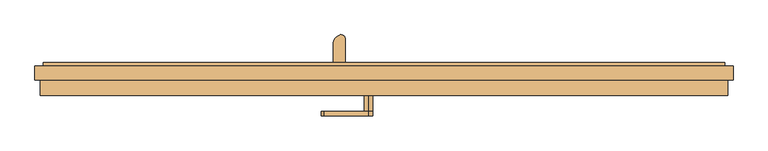
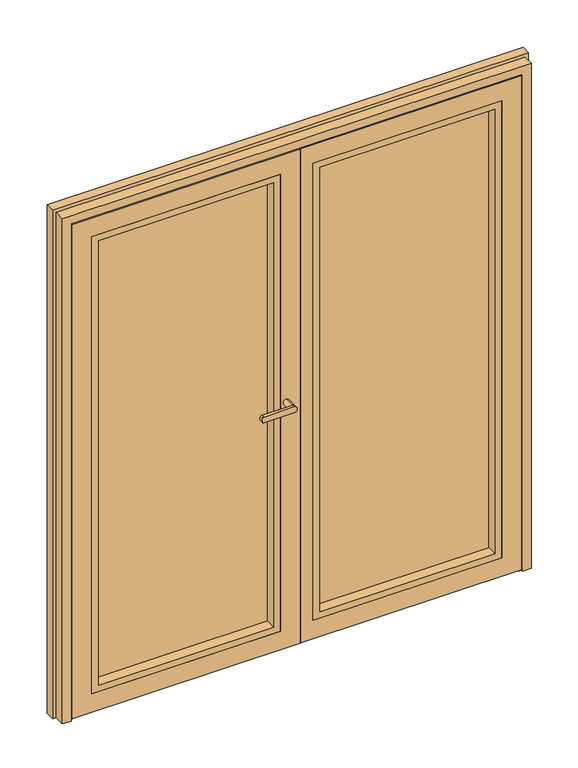
"""IFC4 building model written with IfcOpenShell, lengths in millimetres: door geometry, Schueco_FWS_ADS-90-SI_inw_Family-02 : FWS SI insert unit."""

import ifcopenshell
import ifcopenshell.guid

model = None  # the IFC model being written
_history = None  # IfcOwnerHistory: only IFC2X3 demands one
_inside = {}  # id of a spatial element -> (the spatial element, [elements in it])
_under = {}  # id of a project, library or spatial element -> (it, [spatial elements below it])
_declared = {}  # id of a project -> (the project, [libraries it declares])
_typed = {}  # id of a type object -> (the type object, [elements of that type])
_made_of = {}  # id of a material, layer set ... -> (it, [elements and type objects made of it])


def new_model(schema):
    """Start an empty IFC model of exactly this schema.

    Asked for "IFC4X3", IfcOpenShell would pick the latest addendum, in which some entities
    have other attributes; the version numbers below select the first issue.
    IFC2X3 requires an IfcOwnerHistory on every rooted entity: one is made here for all.
    """
    global model, _history
    if schema == "IFC4X3":
        model = ifcopenshell.file(schema_version=(4, 3, 0, 0))
    else:
        model = ifcopenshell.file(schema=schema)
    _inside.clear()
    _under.clear()
    _declared.clear()
    _typed.clear()
    _made_of.clear()
    _history = None
    if model.schema == "IFC2X3":
        org = make("IfcOrganization", Name="unknown")
        user = make(
            "IfcPersonAndOrganization",
            ThePerson=make("IfcPerson", FamilyName="unknown"),
            TheOrganization=org,
        )
        app = make(
            "IfcApplication",
            ApplicationDeveloper=org,
            Version="unknown",
            ApplicationFullName="unknown",
            ApplicationIdentifier="unknown",
        )
        _history = make(
            "IfcOwnerHistory",
            OwningUser=user,
            OwningApplication=app,
            ChangeAction="ADDED",
            CreationDate=0,
        )
    return model


def make(cls, **values):
    """One entity of the class cls with the attributes given. An attribute that is None is left unset."""
    return model.create_entity(
        cls, **{name: value for name, value in values.items() if value is not None}
    )


def rooted(cls, **values):
    """An entity with a GlobalId (a new one), such as an element, a storey or a relation."""
    return make(cls, GlobalId=ifcopenshell.guid.new(), OwnerHistory=_history, **values)


def si_unit(unit_type, name, prefix=None):
    """IfcSIUnit, for example si_unit("LENGTHUNIT", "METRE", prefix="MILLI")."""
    return make("IfcSIUnit", UnitType=unit_type, Prefix=prefix, Name=name)


def assignment(units):
    """IfcUnitAssignment: the units of a project."""
    return None if units is None else make("IfcUnitAssignment", Units=units)


def point(xyz):
    """IfcCartesianPoint."""
    return None if xyz is None else make("IfcCartesianPoint", Coordinates=xyz)


def direction(xyz):
    """IfcDirection."""
    return None if xyz is None else make("IfcDirection", DirectionRatios=xyz)


def frame(location, z_axis=None, x_axis=None):
    """IfcAxis2Placement3D, a coordinate frame: its origin and axes. An axis left out is left unset."""
    return make(
        "IfcAxis2Placement3D",
        Location=point(location),
        Axis=direction(z_axis),
        RefDirection=direction(x_axis),
    )


def frame_2d(location, x_axis=None):
    """IfcAxis2Placement2D, a coordinate frame in the plane: its origin and x axis."""
    return make(
        "IfcAxis2Placement2D", Location=point(location), RefDirection=direction(x_axis)
    )


def origin():
    """The frame at (0, 0, 0) with its axes left unset."""
    return frame((0.0, 0.0, 0.0))


def place(relative_to, where):
    """IfcLocalPlacement: puts the frame where relative to a parent placement (None: the world)."""
    return make(
        "IfcLocalPlacement", PlacementRelTo=relative_to, RelativePlacement=where
    )


def context(
    kind, dimensions, precision=None, world=None, true_north=None, identifier=None
):
    """IfcGeometricRepresentationContext, for example the 3D "Model" context."""
    return make(
        "IfcGeometricRepresentationContext",
        ContextIdentifier=identifier,
        ContextType=kind,
        CoordinateSpaceDimension=dimensions,
        Precision=precision,
        WorldCoordinateSystem=world,
        TrueNorth=true_north,
    )


def project(units=None, contexts=None):
    """IfcProject with its units and contexts."""
    return rooted(
        "IfcProject",
        Name="project",
        RepresentationContexts=contexts,
        UnitsInContext=assignment(units),
    )


def spatial(cls, under=None, at=None, **own):
    """A site, building, storey or space (cls), placed at a placement, below another one or the project."""
    s = rooted(cls, ObjectPlacement=at, **own)
    if under is not None:
        _under.setdefault(under.id(), (under, []))[1].append(s)
    return s


def polyline(points):
    """IfcPolyline through the points."""
    return make("IfcPolyline", Points=[point(p) for p in points])


def circle_curve(where, radius):
    """IfcCircle in the frame where."""
    return make("IfcCircle", Position=where, Radius=radius)


def ellipse_curve(where, semi_axis1, semi_axis2):
    """IfcEllipse in the frame where."""
    return make(
        "IfcEllipse", Position=where, SemiAxis1=semi_axis1, SemiAxis2=semi_axis2
    )


def trimmed(basis, trim1, trim2, sense, master):
    """IfcTrimmedCurve: the piece of a basis curve between two trims."""
    return make(
        "IfcTrimmedCurve",
        BasisCurve=basis,
        Trim1=trim1,
        Trim2=trim2,
        SenseAgreement=sense,
        MasterRepresentation=master,
    )


def segment(curve, same_sense, transition):
    """IfcCompositeCurveSegment."""
    return make(
        "IfcCompositeCurveSegment",
        Transition=transition,
        SameSense=same_sense,
        ParentCurve=curve,
    )


def composite_curve(segments, self_intersect=None):
    """IfcCompositeCurve: segments joined end to end."""
    return make("IfcCompositeCurve", Segments=segments, SelfIntersect=self_intersect)


def outline(outer, holes=None, kind="AREA"):
    """IfcArbitraryClosedProfileDef: a profile drawn as a closed curve; with holes, ...WithVoids."""
    if holes is None:
        return make("IfcArbitraryClosedProfileDef", ProfileType=kind, OuterCurve=outer)
    return make(
        "IfcArbitraryProfileDefWithVoids",
        ProfileType=kind,
        OuterCurve=outer,
        InnerCurves=holes,
    )


def extrude(swept, where, along, depth):
    """IfcExtrudedAreaSolid: the profile swept, set in the frame where, extruded along a direction by depth."""
    return make(
        "IfcExtrudedAreaSolid",
        SweptArea=swept,
        Position=where,
        ExtrudedDirection=direction(along),
        Depth=depth,
    )


def faces_of(points, faces, orient=None, outer=None):
    """IfcFace entities. A face is a list of loops; a loop is a list of indices into points, from 0.

    orient and outer hold one flag for each loop. By default every Orientation is true, the
    first loop of a face is its IfcFaceOuterBound and the others are IfcFaceBound.
    """
    made = []
    for i, loops in enumerate(faces):
        bounds = []
        for j, loop in enumerate(loops):
            is_outer = j == 0 if outer is None else outer[i][j]
            bounds.append(
                make(
                    "IfcFaceOuterBound" if is_outer else "IfcFaceBound",
                    Bound=make("IfcPolyLoop", Polygon=[points[k] for k in loop]),
                    Orientation=True if orient is None else orient[i][j],
                )
            )
        made.append(make("IfcFace", Bounds=bounds))
    return made


def faceted_brep(points, faces, orient=None, outer=None, voids=None):
    """IfcFacetedBrep: a solid bounded by flat faces; with voids (closed shells), ...WithVoids."""
    shared = [point(p) for p in points]
    hull = make("IfcClosedShell", CfsFaces=faces_of(shared, faces, orient, outer))
    if voids is None:
        return make("IfcFacetedBrep", Outer=hull)
    return make(
        "IfcFacetedBrepWithVoids",
        Outer=hull,
        Voids=[
            make(cls, CfsFaces=faces_of(shared, fs, o, b)) for cls, fs, o, b in voids
        ],
    )


def shape(context_of_items, identifier, shape_type, items):
    """IfcShapeRepresentation: the items that make up one representation, for example the "Body"."""
    return make(
        "IfcShapeRepresentation",
        ContextOfItems=context_of_items,
        RepresentationIdentifier=identifier,
        RepresentationType=shape_type,
        Items=items,
    )


def source(mapping_origin, context_of_items, identifier, shape_type, items):
    """IfcRepresentationMap: a shape defined once, which mapped items show again and again."""
    return make(
        "IfcRepresentationMap",
        MappingOrigin=mapping_origin,
        MappedRepresentation=shape(context_of_items, identifier, shape_type, items),
    )


def transform(
    local_origin,
    x_axis=None,
    y_axis=None,
    z_axis=None,
    scale=None,
    scale2=None,
    scale3=None,
    uniform=True,
):
    """IfcCartesianTransformationOperator3D, or its non-uniform kind. x_axis, y_axis, z_axis: its Axis1, 2, 3."""
    if uniform:
        return make(
            "IfcCartesianTransformationOperator3D",
            Axis1=direction(x_axis),
            Axis2=direction(y_axis),
            LocalOrigin=point(local_origin),
            Scale=scale,
            Axis3=direction(z_axis),
        )
    return make(
        "IfcCartesianTransformationOperator3DnonUniform",
        Axis1=direction(x_axis),
        Axis2=direction(y_axis),
        LocalOrigin=point(local_origin),
        Scale=scale,
        Axis3=direction(z_axis),
        Scale2=scale2,
        Scale3=scale3,
    )


def mapped(mapping_source, mapping_target):
    """IfcMappedItem: shows the shape of a source again, moved by a transform."""
    return make(
        "IfcMappedItem", MappingSource=mapping_source, MappingTarget=mapping_target
    )


def made_of(thing, what):
    """Note that an element or type object is made of a material, layer set ...; save() writes the relation."""
    if what is not None:
        _made_of.setdefault(what.id(), (what, []))[1].append(thing)
    return thing


def element(
    cls,
    number,
    at=None,
    inside=None,
    cuts=None,
    type_object=None,
    material=None,
    context=None,
    identifier="Body",
    shape_type=None,
    held_by="IfcProductDefinitionShape",
    body=None,
    shapes=None,
    **own,
):
    """One element of the class cls, such as IfcWall. Its Tag is "e" and its number.

    at: its placement. inside: the storey or other place that contains it. cuts: it is an
    opening in that element (IfcRelVoidsElement). A single representation is given by context,
    identifier, shape_type and body (its items); several are given by shapes. held_by: the class
    of the entity that holds the representations. save() writes the other relations.
    """
    e = rooted(cls, Tag="e%d" % number, ObjectPlacement=at, **own)
    if body is not None:
        shapes = [shape(context, identifier, shape_type, body)]
    if shapes is not None:
        e.Representation = make(held_by, Representations=shapes)
    if inside is not None:
        _inside.setdefault(inside.id(), (inside, []))[1].append(e)
    if cuts is not None:
        rooted(
            "IfcRelVoidsElement", RelatingBuildingElement=cuts, RelatedOpeningElement=e
        )
    if type_object is not None:
        _typed.setdefault(type_object.id(), (type_object, []))[1].append(e)
    return made_of(e, material)


def aggregate(whole, parts):
    """IfcRelAggregates: a whole, such as a stair, and the parts it consists of."""
    return rooted("IfcRelAggregates", RelatingObject=whole, RelatedObjects=parts)


def save(model, path):
    """Write the relations noted so far, then the file.

    IfcRelAggregates (storeys below a building ...), IfcRelContainedInSpatialStructure (elements
    in a storey), IfcRelDefinesByType, IfcRelAssociatesMaterial and IfcRelDeclares: one each for
    every whole, place, type object, material and project.
    """
    for whole, parts in _under.values():
        aggregate(whole, parts)
    for where, things in _inside.values():
        rooted(
            "IfcRelContainedInSpatialStructure",
            RelatedElements=things,
            RelatingStructure=where,
        )
    for kind, things in _typed.values():
        rooted("IfcRelDefinesByType", RelatedObjects=things, RelatingType=kind)
    for what, things in _made_of.values():
        rooted("IfcRelAssociatesMaterial", RelatedObjects=things, RelatingMaterial=what)
    for by, libraries in _declared.values():
        rooted("IfcRelDeclares", RelatingContext=by, RelatedDefinitions=libraries)
    model.write(path)


def plane_surface(at):
    """IfcPlane: the flat surface through the origin of the frame at, square to its z axis."""
    return make("IfcPlane", Position=at)


def cylinder_surface(at, radius):
    """IfcCylindricalSurface: all points at the distance radius from the z axis of the frame at."""
    return make("IfcCylindricalSurface", Position=at, Radius=radius)


def extruded_surface(curve, direction_of_extrusion, depth):
    """IfcSurfaceOfLinearExtrusion: the curve pushed along a direction by depth."""
    return make(
        "IfcSurfaceOfLinearExtrusion",
        SweptCurve=make("IfcArbitraryOpenProfileDef", ProfileType="CURVE", Curve=curve),
        ExtrudedDirection=direction(direction_of_extrusion),
        Depth=depth,
    )


def advanced_brep(points, edges, surfaces, faces):
    """IfcAdvancedBrep: a solid bounded by faces that lie on surfaces and meet in shared edges.

    An edge is (start, end): straight between two places in points (the first is 0);
    or (start, end, curve); or (start, end, curve, False) where it runs against its curve.
    A face is (place in surfaces, loops), or (place, loops, False) where it looks against
    its surface's normal. A loop lists edges by number (the first is 1), with a minus sign
    where the edge is run from its end to its start. The first loop is the outer one.
    """
    corners = [point(p) for p in points]
    vertices = [make("IfcVertexPoint", VertexGeometry=c) for c in corners]
    made = []
    for start, end, *more in edges:
        made.append(
            make(
                "IfcEdgeCurve",
                EdgeStart=vertices[start],
                EdgeEnd=vertices[end],
                EdgeGeometry=more[0] if more else make("IfcPolyline", Points=[corners[start], corners[end]]),
                SameSense=more[1] if len(more) > 1 else True,
            )
        )
    hull = []
    for where, loops, *sense in faces:
        bounds = []
        for j, loop in enumerate(loops):
            ring = [make("IfcOrientedEdge", EdgeElement=made[abs(k) - 1], Orientation=k > 0) for k in loop]
            bounds.append(
                make(
                    "IfcFaceOuterBound" if j == 0 else "IfcFaceBound",
                    Bound=make("IfcEdgeLoop", EdgeList=ring),
                    Orientation=True,
                )
            )
        hull.append(make("IfcAdvancedFace", Bounds=bounds, FaceSurface=surfaces[where], SameSense=sense[0] if sense else True))
    return make("IfcAdvancedBrep", Outer=make("IfcClosedShell", CfsFaces=hull))


def door_dfdb5275(model_context):
    return source(origin(), model_context, "Body", "SolidModel", [
        faceted_brep([(900.0, -72.5000065, 8.0), (900.0, -72.5000065, 2100.0), (900.0, -81.0002823, 2100.0), (900.0, -81.0002823, 8.0), (17.5, -81.0002823, 8.0), (17.5, -72.5000065, 8.0), (17.5, -72.5000065, 23.0), (885.0, -72.5000065, 23.0), (885.0, -72.5000065, 2085.0), (17.5, -72.5000065, 2085.0), (17.5, -72.5000065, 2100.0), (17.5, -81.0002823, 2100.0), (65.5, -81.0002823, 86.0), (65.5, -81.0002823, 2022.0), (822.0, -81.0002823, 2022.0), (822.0, -81.0002823, 86.0), (822.0, 0.4997603, 2022.0), (822.0, 0.4997603, 86.0), (65.5, 0.4997603, 86.0), (65.5, 0.4997603, 2022.0), (90.5, 0.4997603, 111.0), (90.5, 0.4997603, 1997.0), (797.0, 0.4997603, 1997.0), (797.0, 0.4997603, 111.0), (797.0, 8.9997177, 1997.0), (797.0, 8.9997177, 111.0), (90.5, 8.9997177, 111.0), (90.5, 8.9997177, 1997.0), (870.0, 8.9997177, 38.0), (-12.5, 8.9997177, 38.0), (-12.5, 8.9997177, 2070.0), (870.0, 8.9997177, 2070.0), (870.0, 0.4997603, 2070.0), (870.0, 0.4997603, 38.0), (2.5, 0.4997603, 38.0), (-12.5, 0.4997603, 38.0), (2.5, 0.4997603, 23.0), (2.5, 0.4997603, 2070.0), (2.5, 0.4997603, 2085.0), (885.0, 0.4997603, 2085.0), (885.0, 0.4997603, 23.0), (2.5, -72.5000065, 23.0), (2.5, -72.5000065, 2085.0), (-12.5, 0.4997603, 2070.0)], [[[0, 1, 2, 3]], [[3, 4, 5, 0]], [[0, 5, 6, 7, 8, 9, 10, 1]], [[2, 11, 4, 3], [12, 13, 14, 15]], [[15, 14, 16, 17]], [[17, 18, 12, 15]], [[18, 19, 13, 12]], [[17, 16, 19, 18], [20, 21, 22, 23]], [[23, 22, 24, 25]], [[25, 26, 20, 23]], [[26, 27, 21, 20]], [[28, 29, 30, 31], [25, 24, 27, 26]], [[28, 31, 32, 33]], [[33, 34, 35, 29, 28]], [[36, 34, 33, 32, 37, 38, 39, 40]], [[40, 39, 8, 7]], [[7, 6, 41, 36, 40]], [[41, 42, 38, 37, 34, 36]], [[1, 10, 11, 2]], [[19, 16, 14, 13]], [[27, 24, 22, 21]], [[31, 30, 43, 37, 32]], [[42, 9, 8, 39, 38]], [[6, 5, 4, 11, 10, 9]], [[35, 43, 30, 29]], [[35, 34, 37, 43]], [[9, 42, 41, 6]]]),
        extrude(outline(polyline([(86.0, 65.5), (86.0, 822.0), (2022.0, 822.0), (2022.0, 65.5), (86.0, 65.5)]), holes=[polyline([(113.0, 795.0), (113.0, 92.5), (1995.0, 92.5), (1995.0, 795.0), (113.0, 795.0)])]), frame((0.0, -81.0002823, 0.0), z_axis=(0.0, 1.0, 0.0), x_axis=(0.0, 0.0, 1.0)), (0.0, 0.0, 1.0), 43.5000426),
        extrude(outline(polyline([(65.5, -37.5002397), (65.5, 0.4997603), (822.0, 0.4997603), (822.0, -37.5002397), (65.5, -37.5002397)])), frame((0.0, 0.0, 86.0), z_axis=(0.0, 0.0, 1.0), x_axis=(1.0, 0.0, 0.0)), (0.0, 0.0, 1.0), 1936.0),
        extrude(outline(polyline([(870.0, 0.4997603), (-12.5, 0.4997603), (-12.5, 8.9997177), (870.0, 8.9997177), (870.0, 0.4997603)])), frame((0.0, 0.0, 8.0), z_axis=(0.0, 0.0, 1.0), x_axis=(1.0, 0.0, 0.0)), (0.0, 0.0, 1.0), 30.0),
        extrude(outline(composite_curve([segment(polyline([(-20.8439358, 23.0), (-20.8439358, 4.2956275)]), True, "CONTINUOUS"), segment(trimmed(circle_curve(frame_2d((-31.496302, 15.355415)), 15.3555139), [point((-20.8439358, 4.2956275))], [point((-42.1486683, 4.2956275))], False, "CARTESIAN"), True, "CONTINUOUS"), segment(polyline([(-42.1486683, 4.2956275), (-42.1486683, 23.0), (-20.8439358, 23.0)]), True, "CONTINUOUS")], self_intersect=False)), frame((2.5, 0.0, 0.0), z_axis=(1.0, 0.0, 0.0), x_axis=(0.0, 1.0, 0.0)), (0.0, 0.0, 1.0), 882.5),
        extrude(outline(composite_curve([segment(polyline([(-139.1673236, 8.9997177), (-139.1673236, 59.1618682)]), True, "CONTINUOUS"), segment(trimmed(circle_curve(frame_2d((-111.9889059, 59.1618682)), 27.1784177), [point((-139.1673236, 59.1618682))], [point((-121.5260015, 84.6120194))], False, "CARTESIAN"), True, "CONTINUOUS"), segment(trimmed(circle_curve(frame_2d((-117.4485005, 73.7310321)), 11.6198924), [point((-121.5260015, 84.6120194))], [point((-105.8286081, 73.7310321))], False, "CARTESIAN"), True, "CONTINUOUS"), segment(polyline([(-105.8286081, 73.7310321), (-105.8286081, 8.9997177), (-139.1673236, 8.9997177)]), True, "CONTINUOUS")], self_intersect=False)), frame((0.0, 0.0, 2043.9340013), z_axis=(0.0, 0.0, 1.0), x_axis=(1.0, 0.0, 0.0)), (0.0, 0.0, 1.0), 4.0),
        extrude(outline(polyline([(-139.1673236, 12.9997177), (-105.8286081, 12.9997177), (-105.8286081, 8.9997177), (-139.1673236, 8.9997177), (-139.1673236, 12.9997177)])), frame((0.0, 0.0, 2013.9340013), z_axis=(0.0, 0.0, 1.0), x_axis=(1.0, 0.0, 0.0)), (0.0, 0.0, 1.0), 30.0),
        extrude(outline(polyline([(-139.1673236, 12.9997177), (-105.8286081, 12.9997177), (-105.8286081, 8.9997177), (-139.1673236, 8.9997177), (-139.1673236, 12.9997177)])), frame((0.0, 0.0, 56.9340013), z_axis=(0.0, 0.0, 1.0), x_axis=(1.0, 0.0, 0.0)), (0.0, 0.0, 1.0), 30.0),
        extrude(outline(composite_curve([segment(polyline([(-139.1673236, 8.9997177), (-139.1673236, 59.1618682)]), True, "CONTINUOUS"), segment(trimmed(circle_curve(frame_2d((-111.9889059, 59.1618682)), 27.1784177), [point((-139.1673236, 59.1618682))], [point((-121.5260015, 84.6120194))], False, "CARTESIAN"), True, "CONTINUOUS"), segment(trimmed(circle_curve(frame_2d((-117.4485005, 73.7310321)), 11.6198924), [point((-121.5260015, 84.6120194))], [point((-105.8286081, 73.7310321))], False, "CARTESIAN"), True, "CONTINUOUS"), segment(polyline([(-105.8286081, 73.7310321), (-105.8286081, 8.9997177), (-139.1673236, 8.9997177)]), True, "CONTINUOUS")], self_intersect=False)), frame((0.0, 0.0, 52.9340013), z_axis=(0.0, 0.0, 1.0), x_axis=(1.0, 0.0, 0.0)), (0.0, 0.0, 1.0), 4.0),
        advanced_brep(
        [(-109.782924, 57.5977179, 2043.9340013), (-135.217076, 72.2821425, 2043.9340013), (-109.782924, 57.5977179, 56.9340013), (-135.217076, 72.2821425, 56.9340013)],
        [
            (0, 1, ellipse_curve(frame((-122.5, 64.9399302, 2043.9340013), z_axis=(0.0, 0.0, 1.0), x_axis=(0.5000002582658957, 0.866025254674503, 0.0)), 21.5840887, 14.6844171)),
            (1, 0, ellipse_curve(frame((-122.5, 64.9399302, 2043.9340013), z_axis=(0.0, 0.0, 1.0), x_axis=(0.5000002582658957, 0.866025254674503, 0.0)), 21.5840887, 14.6844171)),
            (2, 3, ellipse_curve(frame((-122.5, 64.9399302, 56.9340013), z_axis=(0.0, 0.0, -1.0), x_axis=(-0.866025254674503, 0.5000002582658957, 0.0)), 14.6844171, 21.5840887)),
            (3, 2, ellipse_curve(frame((-122.5, 64.9399302, 56.9340013), z_axis=(0.0, 0.0, -1.0), x_axis=(-0.866025254674503, 0.5000002582658957, 0.0)), 14.6844171, 21.5840887)),
            (0, 2),
            (3, 1),
        ],
        [
            plane_surface(frame((-135.217076, 72.2821425, 2043.9340013), z_axis=(0.0, 0.0, 1.0), x_axis=(0.5000002582658957, 0.866025254674503, 0.0))),
            plane_surface(frame((-135.217076, 72.2821425, 56.9340013), z_axis=(0.0, 0.0, -1.0), x_axis=(-0.5000002582658957, -0.866025254674503, 0.0))),
            extruded_surface(trimmed(ellipse_curve(frame((-122.5, 64.9399302, 56.9340013), z_axis=(0.0, 0.0, -1.0), x_axis=(-0.866025254674503, 0.5000002582658957, 0.0)), 14.6844171, 21.5840887), [point((-135.217076, 72.2821425, 56.9340013))], [point((-109.782924, 57.5977179, 56.9340013))], True, "CARTESIAN"), (0.0, 0.0, -1987.0), 1987.0),
            extruded_surface(trimmed(ellipse_curve(frame((-122.5, 64.9399302, 56.9340013), z_axis=(0.0, 0.0, -1.0), x_axis=(-0.866025254674503, 0.5000002582658957, 0.0)), 14.6844171, 21.5840887), [point((-109.782924, 57.5977179, 56.9340013))], [point((-135.217076, 72.2821425, 56.9340013))], True, "CARTESIAN"), (0.0, 0.0, -1987.0), 1987.0),
        ],
        [
            (0, [[1, 2]]),
            (1, [[3, 4]]),
            (2, [[5, -4, 6, -1]]),
            (3, [[-6, -3, -5, -2]]),
        ],
    ),
        advanced_brep(
        [(-42.5, -137.0002518, 1038.0113692), (-42.5, -137.0002518, 1061.9886308), (-164.1617926, -137.0002518, 1061.9886308), (-164.1617926, -137.0002518, 1038.0113692), (-42.5, -124.5001648, 1061.9886308), (-42.5, -124.5001648, 1038.0113692), (-164.1617926, -124.5001648, 1038.0113692), (-164.1617926, -124.5001648, 1061.9886308), (-42.5, -81.0002823, 1038.0113692), (-42.5, -81.0002823, 1061.9886308)],
        [
            (0, 1, circle_curve(frame((-42.5, -137.0002518, 1050.0), z_axis=(0.0, -1.0, 0.0), x_axis=(0.0, 0.0, 1.0)), 11.9886308)),
            (1, 2),
            (2, 3, ellipse_curve(frame((-164.1617926, -137.0002518, 1050.0), z_axis=(0.0, -1.0, 0.0), x_axis=(0.0, 0.0, -1.0)), 11.9886308, 7.9050795)),
            (3, 0),
            (4, 5, circle_curve(frame((-42.5, -124.5001648, 1050.0), z_axis=(0.0, -1.0, 0.0), x_axis=(0.0, 0.0, 1.0)), 11.9886308)),
            (5, 6),
            (6, 7, ellipse_curve(frame((-164.1617926, -124.5001648, 1050.0), z_axis=(0.0, 1.0, 0.0), x_axis=(0.0, 0.0, -1.0)), 11.9886308, 7.9050795)),
            (7, 4),
            (3, 6),
            (5, 0),
            (2, 7),
            (1, 4),
            (5, 4, circle_curve(frame((-42.5, -124.5001648, 1050.0), z_axis=(0.0, -1.0, 0.0), x_axis=(0.0, 0.0, 1.0)), 11.9886308)),
            (8, 9, circle_curve(frame((-42.5, -81.0002823, 1050.0), z_axis=(0.0, 1.0, 0.0), x_axis=(0.0, 0.0, 1.0)), 11.9886308)),
            (9, 8, circle_curve(frame((-42.5, -81.0002823, 1050.0), z_axis=(0.0, 1.0, 0.0), x_axis=(0.0, 0.0, 1.0)), 11.9886308)),
            (8, 5),
            (4, 9),
        ],
        [
            plane_surface(frame((-164.1617926, -137.0002518, 1038.0113692), z_axis=(0.0, -1.0, 0.0), x_axis=(-1.0, 0.0, 0.0))),
            plane_surface(frame((-164.1617926, -124.5001648, 1038.0113692), z_axis=(0.0, 1.0, 0.0), x_axis=(1.0, 0.0, 0.0))),
            plane_surface(frame((-42.5, -137.0002518, 1038.0113692), z_axis=(0.0, 0.0, -1.0), x_axis=(0.0, 1.0, 0.0))),
            extruded_surface(trimmed(ellipse_curve(frame((-164.1617926, -124.5001648, 1050.0), z_axis=(0.0, 1.0, 0.0), x_axis=(0.0, 0.0, -1.0)), 11.9886308, 7.9050795), [point((-164.1617926, -124.5001648, 1038.0113692))], [point((-164.1617926, -124.5001648, 1061.9886308))], True, "CARTESIAN"), (0.0, 12.500086999999994, 0.0), 12.500086999999994),
            plane_surface(frame((-164.1617926, -137.0002518, 1061.9886308), z_axis=(0.0, 0.0, 1.0), x_axis=(0.0, 1.0, 0.0))),
            cylinder_surface(frame((-42.5, -124.5001648, 1050.0), z_axis=(0.0, -1.0, 0.0), x_axis=(0.0, 0.0, 1.0)), 11.9886308),
            plane_surface(frame((-42.5, -81.0002823, 1061.9886308), z_axis=(0.0, 1.0, 0.0), x_axis=(-1.0, 0.0, 0.0))),
            cylinder_surface(frame((-42.5, -81.0002823, 1050.0), z_axis=(0.0, -1.0, 0.0), x_axis=(0.0, 0.0, 1.0)), 11.9886308),
        ],
        [
            (0, [[1, 2, 3, 4]]),
            (1, [[5, 6, 7, 8]]),
            (2, [[9, -6, 10, -4]]),
            (3, [[11, -7, -9, -3]]),
            (4, [[12, -8, -11, -2]]),
            (5, [[-10, 13, -12, -1]]),
            (6, [[14, 15]]),
            (7, [[16, -5, 17, -14]]),
            (7, [[-17, -13, -16, -15]]),
        ],
    ),
        faceted_brep([(-900.0, -72.5000065, 8.0), (-900.0, -81.0002823, 8.0), (-900.0, -81.0002823, 2100.0), (-900.0, -72.5000065, 2100.0), (12.5, -72.5000065, 8.0), (12.5, -81.0002823, 8.0), (12.5, -72.5000065, 2100.0), (-885.0, -72.5000065, 23.0), (-2.5, -72.5000065, 23.0), (-2.5, -72.5000065, 2085.0), (-885.0, -72.5000065, 2085.0), (12.5, -81.0002823, 2100.0), (-65.5, -81.0002823, 86.0), (-822.0, -81.0002823, 86.0), (-822.0, -81.0002823, 2022.0), (-65.5, -81.0002823, 2022.0), (-822.0, 0.4997603, 86.0), (-822.0, 0.4997603, 2022.0), (-65.5, 0.4997603, 86.0), (-65.5, 0.4997603, 2022.0), (-90.5, 0.4997603, 111.0), (-797.0, 0.4997603, 111.0), (-797.0, 0.4997603, 1997.0), (-90.5, 0.4997603, 1997.0), (-797.0, 8.9997177, 111.0), (-797.0, 8.9997177, 1997.0), (-90.5, 8.9997177, 111.0), (-90.5, 8.9997177, 1997.0), (-17.5, 8.9997177, 2070.0), (-17.5, 8.9997177, 38.0), (-27.5, 8.9997177, 38.0), (-870.0, 8.9997177, 38.0), (-870.0, 8.9997177, 2070.0), (-27.5, 8.9997177, 2070.0), (-870.0, 0.4997603, 38.0), (-870.0, 0.4997603, 2070.0), (-17.5, 0.4997603, 38.0), (-27.5, 0.4997603, 38.0), (-17.5, 0.4997603, 2070.0), (-2.5, 0.4997603, 23.0), (-885.0, 0.4997603, 23.0), (-885.0, 0.4997603, 2085.0), (-2.5, 0.4997603, 2085.0), (-27.5, 0.4997603, 2070.0)], [[[0, 1, 2, 3]], [[1, 0, 4, 5]], [[4, 0, 3, 6], [7, 8, 9, 10]], [[5, 4, 6, 11]], [[1, 5, 11, 2], [12, 13, 14, 15]], [[13, 16, 17, 14]], [[16, 13, 12, 18]], [[18, 12, 15, 19]], [[16, 18, 19, 17], [20, 21, 22, 23]], [[21, 24, 25, 22]], [[24, 21, 20, 26]], [[26, 20, 23, 27]], [[28, 29, 30, 31, 32, 33], [24, 26, 27, 25]], [[31, 34, 35, 32]], [[34, 31, 30, 29, 36, 37]], [[36, 29, 28, 38]], [[39, 40, 41, 42], [36, 38, 43, 35, 34, 37]], [[40, 7, 10, 41]], [[7, 40, 39, 8]], [[8, 39, 42, 9]], [[11, 6, 3, 2]], [[19, 15, 14, 17]], [[27, 23, 22, 25]], [[38, 28, 33, 32, 35, 43]], [[9, 42, 41, 10]]]),
        extrude(outline(polyline([(86.0, -65.5), (2022.0, -65.5), (2022.0, -822.0), (86.0, -822.0), (86.0, -65.5)]), holes=[polyline([(113.0, -795.0), (1995.0, -795.0), (1995.0, -92.5), (113.0, -92.5), (113.0, -795.0)])]), frame((0.0, -81.0002823, 0.0), z_axis=(0.0, 1.0, 0.0), x_axis=(0.0, 0.0, 1.0)), (0.0, 0.0, 1.0), 43.5000426),
        extrude(outline(polyline([(-65.5, -37.5002397), (-822.0, -37.5002397), (-822.0, 0.4997603), (-65.5, 0.4997603), (-65.5, -37.5002397)])), frame((0.0, 0.0, 86.0), z_axis=(0.0, 0.0, 1.0), x_axis=(1.0, 0.0, 0.0)), (0.0, 0.0, 1.0), 1936.0),
        extrude(outline(polyline([(-870.0, 0.4997603), (-870.0, 8.9997177), (-17.5, 8.9997177), (-17.5, 0.4997603), (-870.0, 0.4997603)])), frame((0.0, 0.0, 8.0), z_axis=(0.0, 0.0, 1.0), x_axis=(1.0, 0.0, 0.0)), (0.0, 0.0, 1.0), 30.0),
        extrude(outline(composite_curve([segment(polyline([(-20.8439358, 23.0), (-20.8439358, 4.2956275)]), True, "CONTINUOUS"), segment(trimmed(circle_curve(frame_2d((-31.496302, 15.355415)), 15.3555139), [point((-20.8439358, 4.2956275))], [point((-42.1486683, 4.2956275))], False, "CARTESIAN"), True, "CONTINUOUS"), segment(polyline([(-42.1486683, 4.2956275), (-42.1486683, 23.0), (-20.8439358, 23.0)]), True, "CONTINUOUS")], self_intersect=False)), frame((-885.0, 0.0, 0.0), z_axis=(1.0, 0.0, 0.0), x_axis=(0.0, 1.0, 0.0)), (0.0, 0.0, 1.0), 882.5),
        faceted_brep([(930.999943, 8.9997177, 2130.999943), (930.999943, 0.0, 2130.999943), (930.999943, 0.0, 0.0), (930.999943, 8.9997177, 0.0), (-954.0, 0.0, 0.0), (-954.0, 0.0, 2154.0), (954.0, 0.0, 2154.0), (954.0, 0.0, 0.0), (-930.999943, 0.0, 2130.999943), (-930.999943, 0.0, 0.0), (954.0, -38.0, 0.0), (940.0, -38.0, 0.0), (940.0, -81.0002823, 0.0), (904.9999114, -81.0002823, 0.0), (904.9999114, -72.5000065, 0.0), (893.4999114, -72.5000065, 0.0), (893.4999114, 0.4997603, 0.0), (874.9999888, 0.4997603, 0.0), (874.9999888, 8.9997177, 0.0), (-874.9999888, 8.9997177, 0.0), (-930.999943, 8.9997177, 0.0), (-930.999943, 8.9997177, 2130.999943), (874.9999888, 8.9997177, 2074.9999888), (-874.9999888, 8.9997177, 2074.9999888), (904.9999114, -81.0002823, 2104.9999114), (904.9999114, -72.5000065, 2104.9999114), (-904.9999114, -72.5000065, 0.0), (-893.4999114, -72.5000065, 0.0), (-893.4999114, -72.5000065, 2093.4999114), (893.4999114, -72.5000065, 2093.4999114), (-904.9999114, -72.5000065, 2104.9999114), (-940.0, -81.0002823, 0.0), (-904.9999114, -81.0002823, 0.0), (-904.9999114, -81.0002823, 2104.9999114), (940.0, -81.0002823, 2140.0), (-940.0, -81.0002823, 2140.0), (940.0, -38.0, 2140.0), (-954.0, -38.0, 0.0), (-940.0, -38.0, 0.0), (-940.0, -38.0, 2140.0), (954.0, -38.0, 2154.0), (-954.0, -38.0, 2154.0), (-874.9999888, 0.4997603, 0.0), (-893.4999114, 0.4997603, 0.0), (874.9999888, 0.4997603, 2074.9999888), (-874.9999888, 0.4997603, 2074.9999888), (893.4999114, 0.4997603, 2093.4999114), (-893.4999114, 0.4997603, 2093.4999114)], [[[0, 1, 2, 3]], [[4, 5, 6, 7, 2, 1, 8, 9]], [[3, 2, 7, 10, 11, 12, 13, 14, 15, 16, 17, 18]], [[19, 20, 21, 0, 3, 18, 22, 23]], [[24, 25, 14, 13]], [[26, 27, 28, 29, 15, 14, 25, 30]], [[31, 32, 33, 24, 13, 12, 34, 35]], [[34, 12, 11, 36]], [[37, 38, 39, 36, 11, 10, 40, 41]], [[4, 9, 20, 19, 42, 43, 27, 26, 32, 31, 38, 37]], [[20, 9, 8, 21]], [[18, 17, 44, 22]], [[42, 19, 23, 45]], [[32, 26, 30, 33]], [[31, 35, 39, 38]], [[4, 37, 41, 5]], [[6, 40, 10, 7]], [[43, 42, 45, 44, 17, 16, 46, 47]], [[16, 15, 29, 46]], [[27, 43, 47, 28]], [[21, 8, 1, 0]], [[33, 30, 25, 24]], [[35, 34, 36, 39]], [[23, 22, 44, 45]], [[5, 41, 40, 6]], [[47, 46, 29, 28]]]),
    ])


if __name__ == "__main__":
    model = new_model("IFC4")
    model_context = context("Model", 3, world=origin())
    ifc_project = project(units=[si_unit("LENGTHUNIT", "METRE", prefix="MILLI")], contexts=[model_context])
    site = spatial("IfcSite", under=ifc_project)
    building = spatial("IfcBuilding", under=site)
    placement = place(None, origin())
    door_shape = door_dfdb5275(model_context)
    element("IfcDoor", 1, ObjectType="Schueco_FWS_ADS-90-SI_inw_Family-02 : FWS SI insert unit", at=placement, inside=building, context=model_context, shape_type="MappedRepresentation", body=[
        mapped(door_shape, transform((0.0, 0.0, 0.0), x_axis=(1.0, 0.0, 0.0), y_axis=(0.0, 1.0, 0.0), z_axis=(0.0, 0.0, 1.0))),
    ])
    save(model, "model.ifc")

# Revit data of these elements
# Type "Schueco_FWS_ADS-90-SI_inw_Family-02 : FWS SI insert unit"
#   Type Mark = "57"
#   __NOTE__ = "Data describes the optimum values of the entire system. The properites of a selected design option have to be determined on an individual basis!"
#   Wind load resistance = "Class C3"
#   Watertightness = "Class 7A"
#   Thermal insulation = "Uf = 1.2 W/(m²K)"
#   Sound insulation = "..."
#   Schueco thermal insulation standard = "Highly thermally insulated"
#   Opening type = "Inward-opening, Flush-fitted"
#   Model = "Schueco ADS 90.SI"
#   Mechanical loading = "Class 3"
#   Maximum leaf width in mm = "1400"
#   Maximum leaf weight in kg = "160"
#   Maximum leaf height in mm = "2500"
#   Material = "Aluminium"
#   Long term functionality = "..."
#   Construction Type = "Door, double-leaf, inward-opening"
#   Manufacturer = "Schueco International KG"
#   Glazing data = "Triple glazing 38mm"
#   Façade insert unit = "yes"
#   Family creation date = "08.2017"
#   Description = "Schueco Aluminium Door System (ADS)"
#   Burglar resistance = "Class RC 3"
#   Areas of use = "Public buildings, Side entrance"
#   Analytic Construction = "<None>"
#   Air permeability = "Class 4"
#   Width [instance default] = 1116.773 mm
#   Leaf opening angle [instance default] = 0.00°
#   IOf_T = 38 mm
#   Height [instance default] = 1990.31 mm
#   Glazing area [instance default] = 1.05465 m²
#   F2_W [instance default] = 558.386 mm
#   F1_W [instance default] = 558.386 mm
#   Distance from bottom to handles [instance default] = 1050 mm
#   Clear opening width [instance default] = 958.773 mm
#   Active leaf width = 1100 mm
#   Standard threshold = no
#   Low level threshold = yes
#   Handles = yes
#   All fields of identical width = yes
#   Glass = none
#   Frame = Alu
#   Fittings = none
# Element 1 (IfcDoor, "Schueco_FWS_ADS-90-SI_inw_Family-02 : FWS SI insert unit")
#   Width = 1908 mm
#   Height = 2154 mm
#   Glazing area = 2.64421 m²
#   F2_W = 954 mm
#   F1_W = 954 mm
#   Clear opening width = 1750 mm
#   Materials on its faces: "Alu", "Glass"
# Materials
#   "Alu": class "Glas", colour RGB 140 140 140, transparency 0
#   "Glass": class "Glass", colour RGB 128 128 255, transparency 0.75, Description = "Soda Lime Glass", Cost = 0
